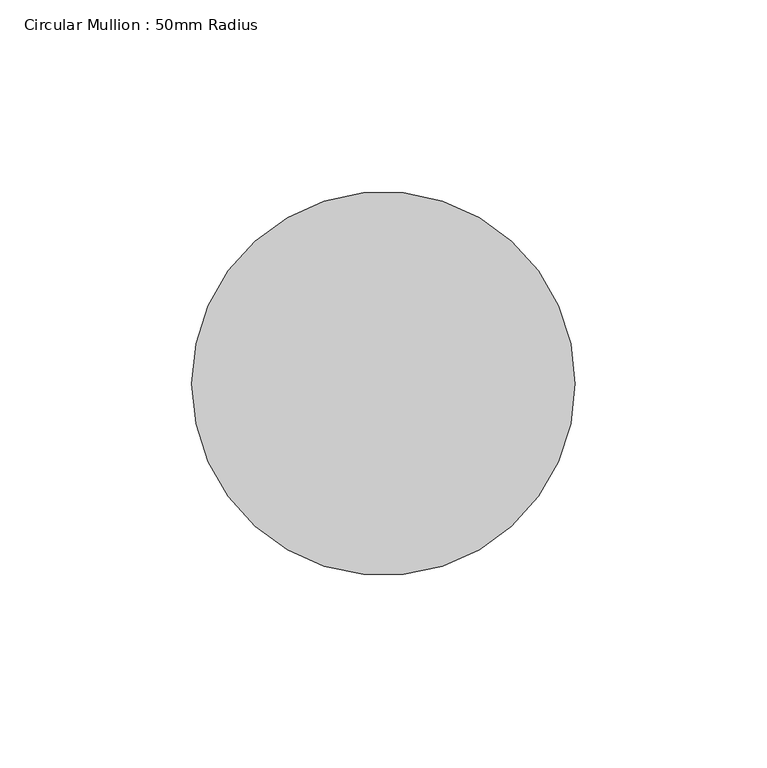
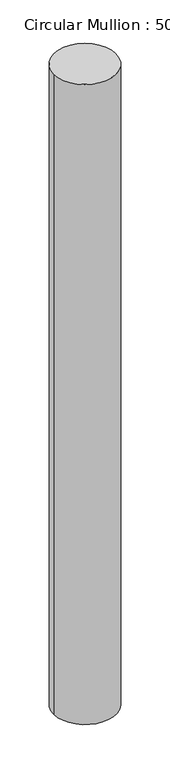
"""IFC4 building model written with IfcOpenShell, lengths in millimetres: member geometry, Circular Mullion : 50mm Radius."""

from ifc_helpers import new_model, si_unit, point, frame, origin, origin_2d, place, context, project, spatial, circle_curve, trimmed, segment, composite_curve, outline, extrude, source, transform, mapped, element, save


def circular_mullion_50mm_radius_f295a4b6(model_context):
    return source(origin(), model_context, "Body", "SweptSolid", [
        extrude(outline(composite_curve([segment(trimmed(circle_curve(origin_2d(), 50.0), [point((50.0, 0.0))], [point((-50.0, 0.0))], False, "CARTESIAN"), True, "CONTINUOUS"), segment(trimmed(circle_curve(origin_2d(), 50.0), [point((-50.0, 0.0))], [point((50.0, 0.0))], False, "CARTESIAN"), True, "CONTINUOUS")], self_intersect=False)), frame((0.0, 0.0, -1089.2569805), z_axis=(0.0, 0.0, 1.0), x_axis=(1.0, 0.0, 0.0)), (0.0, 0.0, 1.0), 1089.2569805),
    ])


if __name__ == "__main__":
    model = new_model("IFC4")
    model_context = context("Model", 3, world=origin())
    ifc_project = project(units=[si_unit("LENGTHUNIT", "METRE", prefix="MILLI")], contexts=[model_context])
    site = spatial("IfcSite", under=ifc_project)
    building = spatial("IfcBuilding", under=site)
    placement = place(None, origin())
    circular_mullion_50mm_radius_shape = circular_mullion_50mm_radius_f295a4b6(model_context)
    element("IfcMember", 1, ObjectType="Circular Mullion : 50mm Radius", at=placement, inside=building, context=model_context, shape_type="MappedRepresentation", body=[
        mapped(circular_mullion_50mm_radius_shape, transform((0.0, 0.0, 0.0), x_axis=(1.0, 0.0, 0.0), y_axis=(0.0, 1.0, 0.0), z_axis=(0.0, 0.0, 1.0))),
    ])
    save(model, "model.ifc")

# Revit data of these elements
# Type "Circular Mullion : 50mm Radius"
#   built-in parameter 1007350 = 0.164042 (stored number, unit not read)
# Element 1 (IfcMember, "Circular Mullion : 50mm Radius")
#   Materials on its faces: "Aluminium"
# Materials
#   "Aluminium": class "Metal", colour RGB 247 247 247, transparency 0, Description = "Aluminium 6061", Cost = 0
